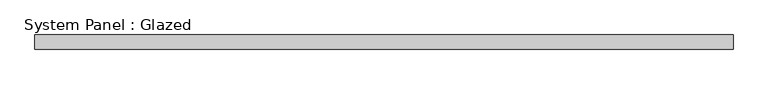
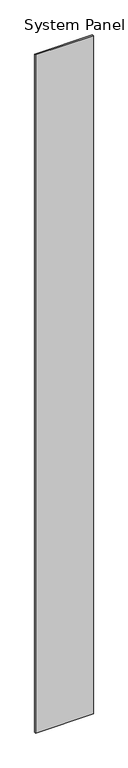
"""IFC4 building model written with IfcOpenShell, lengths in millimetres: plate geometry, System Panel : Glazed."""

from ifc_helpers import new_model, si_unit, origin, origin_with_axes, place, context, project, spatial, polyline, outline, extrude, source, transform, mapped, element, save


def system_panel_glazed_d00c2bb3(model_context):
    return source(origin(), model_context, "Body", "SweptSolid", [
        extrude(outline(polyline([(609.5367635, 19.05), (-609.5367635, 19.05), (-609.5367635, 44.45), (609.5367635, 44.45), (609.5367635, 19.05)])), origin_with_axes(), (0.0, 0.0, 1.0), 15087.6),
    ])


if __name__ == "__main__":
    model = new_model("IFC4")
    model_context = context("Model", 3, world=origin())
    ifc_project = project(units=[si_unit("LENGTHUNIT", "METRE", prefix="MILLI")], contexts=[model_context])
    site = spatial("IfcSite", under=ifc_project)
    building = spatial("IfcBuilding", under=site)
    placement = place(None, origin())
    system_panel_glazed_shape = system_panel_glazed_d00c2bb3(model_context)
    element("IfcPlate", 1, ObjectType="System Panel : Glazed", at=placement, inside=building, context=model_context, shape_type="MappedRepresentation", body=[
        mapped(system_panel_glazed_shape, transform((0.0, 0.0, 0.0), x_axis=(1.0, 0.0, 0.0), y_axis=(0.0, 1.0, 0.0), z_axis=(0.0, 0.0, 1.0))),
    ])
    save(model, "model.ifc")

# Revit data of these elements
# Type "System Panel : Glazed"
#   Construction Type Id = "GSP4R"
#   Analytic Construction = "1/8 in Pilkington single glazing"
#   Visual Light Transmittance = 0.9
#   Solar Heat Gain Coefficient = 0.86
#   Heat Transfer Coefficient (U) = 1.18115 BTU/(h·ft²·°F)
#   Define Thermal Properties by = 1
# Element 1 (IfcPlate, "System Panel : Glazed")
#   Materials on its faces: "Glass"
# Materials
#   "Glass": class "Glass", colour RGB 0 128 192, transparency 0.75, Description = "Soda Lime Glass", Cost = 0
